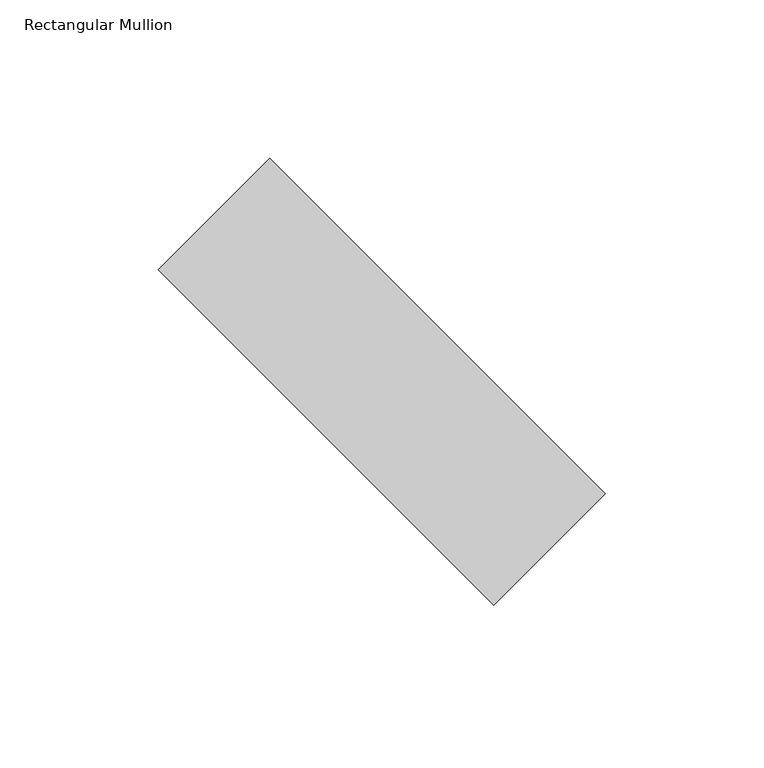
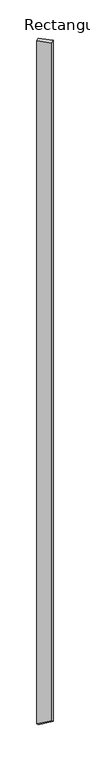
"""IFC4 building model written with IfcOpenShell, lengths in millimetres: member geometry, Rectangular Mullion : tilted mullions."""

from ifc_helpers import new_model, si_unit, origin, place, context, project, spatial, faceted_brep, source, transform, mapped, element, save


def rectangular_mullion_e2a2a6fe(model_context):
    return source(origin(), model_context, "Body", "Brep", [
        faceted_brep([(-35.3553391, 70.7106781, 0.0), (-70.7106781, 35.3553391, 0.0), (35.3553391, -70.7106781, 0.0), (70.7106781, -35.3553391, 0.0), (-35.3553391, 70.7106781, -8054.2512911), (-70.7106781, 35.3553391, -8009.2124229), (35.3553391, -70.7106781, -7944.0702464), (70.7106781, -35.3553391, -7989.1091146)], [[[0, 1, 2, 3]], [[1, 0, 4, 5]], [[2, 1, 5, 6]], [[3, 2, 6, 7]], [[0, 3, 7, 4]], [[4, 7, 6, 5]]]),
    ])


if __name__ == "__main__":
    model = new_model("IFC4")
    model_context = context("Model", 3, world=origin())
    ifc_project = project(units=[si_unit("LENGTHUNIT", "METRE", prefix="MILLI")], contexts=[model_context])
    site = spatial("IfcSite", under=ifc_project)
    building = spatial("IfcBuilding", under=site)
    placement = place(None, origin())
    rectangular_mullion_shape = rectangular_mullion_e2a2a6fe(model_context)
    element("IfcMember", 1, ObjectType="Rectangular Mullion : tilted mullions", at=placement, inside=building, context=model_context, shape_type="MappedRepresentation", body=[
        mapped(rectangular_mullion_shape, transform((0.0, 0.0, 0.0), x_axis=(1.0, 0.0, 0.0), y_axis=(0.0, 1.0, 0.0), z_axis=(0.0, 0.0, 1.0))),
    ])
    save(model, "model.ifc")

# Revit data of these elements
# Type "Rectangular Mullion : tilted mullions"
#   built-in parameter 1007304 = 0.492126 (stored number, unit not read)
#   built-in parameter 1007301 = 0.082021 (stored number, unit not read)
#   built-in parameter 1007300 = 0.082021 (stored number, unit not read)
# Element 1 (IfcMember, "Rectangular Mullion : tilted mullions")
#   Materials on its faces: "Aluminum"
# Materials
#   "Aluminum": class "Metal", colour RGB 244 244 244, transparency 0, Description = "Aluminum 6061", Cost = 0
